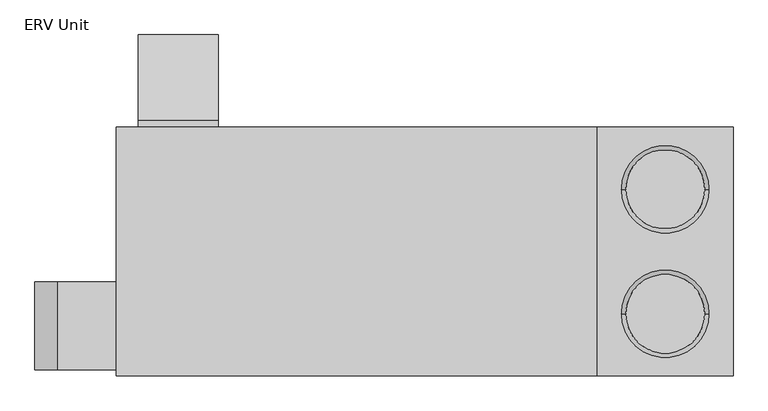
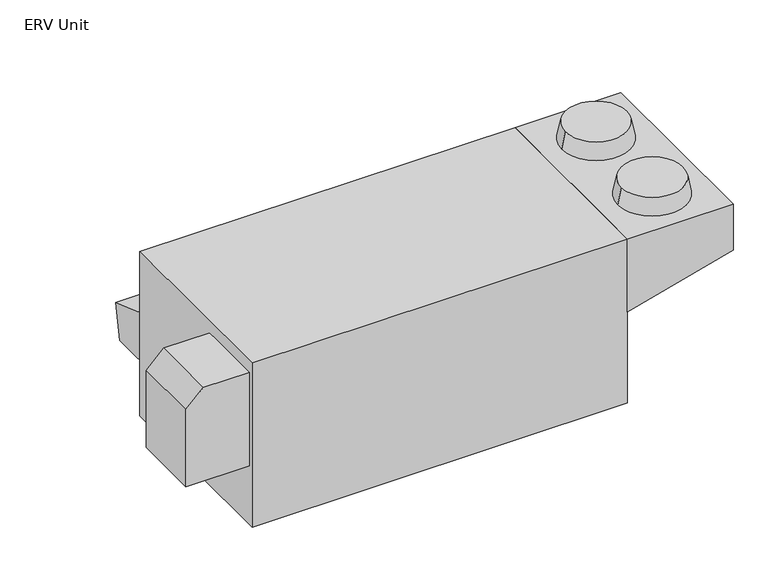
"""IFC4 building model written with IfcOpenShell, lengths in millimetres: proxy geometry, Energy Recovery-ER_H : ERV Unit."""

from ifc_helpers import new_model, si_unit, frame, origin, place, context, project, spatial, polyline, circle_curve, outline, extrude, source, transform, mapped, element, save
from ifc_brep_helpers import plane_surface, revolved_surface, advanced_brep


def erv_unit_62530c4e(model_context):
    return source(origin(), model_context, "Body", "SolidModel", [
        extrude(outline(polyline([(740.0249593, 200.025), (740.0249593, 635.0), (778.1249593, 635.0), (1267.0749593, 463.55), (1216.2749593, 200.025), (740.0249593, 200.025)])), frame((-44.3389519, 0.0, 0.0), z_axis=(1.0, 0.0, 0.0), x_axis=(0.0, 1.0, 0.0)), (0.0, 0.0, 1.0), 457.2),
        advanced_brep(
        [(3188.1285481, -326.7750407, 1346.2), (2736.6435481, -326.7750407, 1346.2), (3213.2110481, -326.7750407, 1219.2), (2711.5610481, -326.7750407, 1219.2)],
        [
            (0, 1, circle_curve(frame((2962.3860481, -326.7750407, 1346.2), z_axis=(0.0, 0.0, 1.0), x_axis=(1.0, 0.0, 0.0)), 225.7425)),
            (1, 0, circle_curve(frame((2962.3860481, -326.7750407, 1346.2), z_axis=(0.0, 0.0, 1.0), x_axis=(-1.0, 0.0, 0.0)), 225.7425)),
            (2, 3, circle_curve(frame((2962.3860481, -326.7750407, 1219.2), z_axis=(0.0, 0.0, -1.0), x_axis=(-1.0, 0.0, 0.0)), 250.825)),
            (3, 2, circle_curve(frame((2962.3860481, -326.7750407, 1219.2), z_axis=(0.0, 0.0, -1.0), x_axis=(1.0, 0.0, 0.0)), 250.825)),
            (3, 1),
            (0, 2),
        ],
        [
            plane_surface(frame((2962.3860481, -326.7750407, 1346.2), z_axis=(0.0, 0.0, 1.0), x_axis=(0.0, 1.0, 0.0))),
            plane_surface(frame((2962.3860481, -326.7750407, 1219.2), z_axis=(0.0, 0.0, -1.0), x_axis=(0.0, 1.0, 0.0))),
            revolved_surface(polyline([(3188.1285481, -326.7750407, 1346.2), (3213.2110481, -326.7750407, 1219.2)]), (2962.3860481, -326.7750407, 2489.2), (0.0, 0.0, -1.0)),
            revolved_surface(polyline([(2736.6435481, -326.7750407, 1346.2), (2711.5610481, -326.7750407, 1219.2)]), (2962.3860481, -326.7750407, 2489.2), (0.0, 0.0, -1.0)),
        ],
        [
            (0, [[1, 2]]),
            (1, [[3, 4]]),
            (2, [[-4, 5, -1, 6]]),
            (3, [[-3, -6, -2, -5]]),
        ],
    ),
        advanced_brep(
        [(3188.1285481, 384.4249593, 1346.2), (2736.6435481, 384.4249593, 1346.2), (3213.2110481, 384.4249593, 1219.2), (2711.5610481, 384.4249593, 1219.2)],
        [
            (0, 1, circle_curve(frame((2962.3860481, 384.4249593, 1346.2), z_axis=(0.0, 0.0, 1.0), x_axis=(1.0, 0.0, 0.0)), 225.7425)),
            (1, 0, circle_curve(frame((2962.3860481, 384.4249593, 1346.2), z_axis=(0.0, 0.0, 1.0), x_axis=(-1.0, 0.0, 0.0)), 225.7425)),
            (2, 3, circle_curve(frame((2962.3860481, 384.4249593, 1219.2), z_axis=(0.0, 0.0, -1.0), x_axis=(-1.0, 0.0, 0.0)), 250.825)),
            (3, 2, circle_curve(frame((2962.3860481, 384.4249593, 1219.2), z_axis=(0.0, 0.0, -1.0), x_axis=(1.0, 0.0, 0.0)), 250.825)),
            (3, 1),
            (0, 2),
        ],
        [
            plane_surface(frame((2962.3860481, 384.4249593, 1346.2), z_axis=(0.0, 0.0, 1.0), x_axis=(0.0, 1.0, 0.0))),
            plane_surface(frame((2962.3860481, 384.4249593, 1219.2), z_axis=(0.0, 0.0, -1.0), x_axis=(0.0, 1.0, 0.0))),
            revolved_surface(polyline([(3188.1285481, 384.4249593, 1346.2), (3213.2110481, 384.4249593, 1219.2)]), (2962.3860481, 384.4249593, 2489.2), (0.0, 0.0, -1.0)),
            revolved_surface(polyline([(2736.6435481, 384.4249593, 1346.2), (2711.5610481, 384.4249593, 1219.2)]), (2962.3860481, 384.4249593, 2489.2), (0.0, 0.0, -1.0)),
        ],
        [
            (0, [[1, 2]]),
            (1, [[3, 4]]),
            (2, [[-4, 5, -1, 6]]),
            (3, [[-3, -6, -2, -5]]),
        ],
    ),
        extrude(outline(polyline([(1219.2, 3349.7360481), (1219.2, 2575.0360481), (654.05, 2575.0360481), (863.6, 3349.7360481), (1219.2, 3349.7360481)])), frame((0.0, -682.3750407, 0.0), z_axis=(0.0, 1.0, 0.0), x_axis=(0.0, 0.0, 1.0)), (0.0, 0.0, 1.0), 1422.4),
        extrude(outline(polyline([(403.225, -171.3389519), (1127.125, -171.3389519), (1127.125, -507.8889519), (1000.125, -634.8889519), (403.225, -634.8889519), (403.225, -171.3389519)])), frame((0.0, -647.4500407, 0.0), z_axis=(0.0, 1.0, 0.0), x_axis=(0.0, 0.0, 1.0)), (0.0, 0.0, 1.0), 501.65),
        extrude(outline(polyline([(2060.6860481, 606.6749593), (2060.6860481, 276.4749593), (1425.6860481, 276.4749593), (1425.6860481, 606.6749593), (2060.6860481, 606.6749593)])), frame((0.0, 0.0, -50.8), z_axis=(0.0, 0.0, 1.0), x_axis=(1.0, 0.0, 0.0)), (0.0, 0.0, 1.0), 3.175),
        extrude(outline(polyline([(2194.0360481, -129.9250407), (2194.0360481, -587.1250407), (1838.4360481, -587.1250407), (1838.4360481, -129.9250407), (2194.0360481, -129.9250407)])), frame((0.0, 0.0, -50.8), z_axis=(0.0, 0.0, 1.0), x_axis=(1.0, 0.0, 0.0)), (0.0, 0.0, 1.0), 3.175),
        extrude(outline(polyline([(2575.0360481, 740.0249593), (2575.0360481, -682.3750407), (-171.3389519, -682.3750407), (-171.3389519, 740.0249593), (2575.0360481, 740.0249593)])), frame((0.0, 0.0, -50.8), z_axis=(0.0, 0.0, 1.0), x_axis=(1.0, 0.0, 0.0)), (0.0, 0.0, 1.0), 1270.0),
    ])


if __name__ == "__main__":
    model = new_model("IFC4")
    model_context = context("Model", 3, world=origin())
    ifc_project = project(units=[si_unit("LENGTHUNIT", "METRE", prefix="MILLI")], contexts=[model_context])
    site = spatial("IfcSite", under=ifc_project)
    building = spatial("IfcBuilding", under=site)
    placement = place(None, origin())
    erv_unit_shape = erv_unit_62530c4e(model_context)
    element("IfcBuildingElementProxy", 1, Name="Energy Recovery-ER_H : ERV Unit", ObjectType="Energy Recovery-ER_H : ERV Unit", at=placement, inside=building, context=model_context, shape_type="MappedRepresentation", body=[
        mapped(erv_unit_shape, transform((0.0, 0.0, 0.0), x_axis=(1.0, 0.0, 0.0), y_axis=(0.0, 1.0, 0.0), z_axis=(0.0, 0.0, 1.0))),
    ])
    save(model, "model.ifc")

# Revit data of these elements
# Type "Energy Recovery-ER_H : ERV Unit"
#   Version Family = "rfa 1.0 Beta"
#   Version Data = "NA"
#   URL = "http://www.greenheck.com/products/detail/51"
#   Tag = ""
#   Supply Filter = ""
#   OAI Weatherhood End Description = "Louvered Outdoor Air Intake"
#   OAI Duct Top Description = "Alternative connector is used"
#   OAI Duct End Description = "Alternative connector is used"
#   OAD Duct Top Description = "Alternative connector is used"
#   OAD Duct Side Description = "Alternative connector is used"
#   OAD Duct End Description = "Alternative connector is used"
#   OAD Duct Bottom Description = "Supply Air Discharge"
#   Model = "ERCH-20M-15"
#   Manufacturing Location = "United States"
#   Manufacturer = "Greenheck"
#   Invalid Connector = "Alternative connector is used"
#   Exhaust Filter = ""
#   Energy Wheel Model = "0"
#   EAI Duct Top Description = "Alternative connector is used"
#   EAI Duct Bottom Description = "Exhaust Air Intake"
#   EAI Duct Back Description = "Alternative connector is used"
#   EAD Weatherhood Side Description = "Side Exhaust Air Weatherhood"
#   EAD Weatherhood End Description = "Alternative connector is used"
#   EAD Duct Top Description = "Alternative connector is used"
#   EAD Duct Side Description = "Alternative connector is used"
#   EAD Duct End Description = "Alternative connector is used"
#   Description = "Energy Recovery with Cooling & Heating"
#   Copyright © = "© Greenheck Fan Corp 2009"
#   Configured Mark Name = "ERV Unit"
#   Voltage = 460 V
#   Unit Weight = 0.0000625 kip
#   Supply Static Pressure = 0.00 in-wg
#   Supply Air Flow Rate = 1400 CFM
#   PDX Length = 774.7 mm
#   PDX Front Height = 355.6 mm
#   PDX Cooling Radius Top = 225.743 mm
#   PDX Cooling Radius = 250.825 mm
#   PDX Back Height = 565.15 mm
#   OAI Half Depth = 231.775 mm
#   OAI Duct Width = 501.65 mm
#   OAI Duct Vert = 815.975 mm
#   OAI Duct Horiz = 285.75 mm
#   OAI Duct Height = 723.9 mm
#   OAI Depth = 463.55 mm
#   OAD Duct Width = 457.2 mm
#   OAD Duct Vert = 558.8 mm
#   OAD Duct Horiz = 323.85 mm
#   OAD Duct Height = 355.6 mm
#   Length PDX = 762 mm
#   IG Heater Width = 787.4 mm
#   IG Heater Offset = 25.4 mm
#   IG Heater Height = 0 mm
#   IG Heater Height NZ = 25.4 mm
#   IG Heater Depth = 254 mm
#   Half Under Sizing = 25.4 mm
#   Exhaust Static Pressure = 0.00 in-wg
#   Exhaust Air Flow Rate = 1400 CFM
#   Energy Wheel Depth = 38.1 mm
#   Electrical Load = 0 VA
#   Electrical Current = 60 Hz
#   EAI Duct Width = 330.2 mm
#   EAI Duct Vert = 831.85 mm
#   EAI Duct Horiz = 298.45 mm
#   EAI Duct Height = 635 mm
#   EAD Duct Width = 457.2 mm
#   EAD Duct Vert = 514.35 mm
#   EAD Duct Horiz = 355.6 mm
#   EAD Duct Height = 434.975 mm
#   EAD Depth = 527.05 mm
#   CurbWidth = 1371.6 mm
#   CurbLength = 2695.575 mm
#   Curb Under Sizing = 50.8 mm
#   Curb Height = 25.4 mm
#   Base Width = 1422.4 mm
#   Base Length = 2746.375 mm
#   Base Height = 1270 mm
#   VFD = no
#   Roof Curb = no
#   Phase = 3
#   Packaged DX = yes
#   OAI Weatherhood End = yes
#   OAI Duct Top = no
#   OAI Duct End = no
#   OAD Duct Top = no
#   OAD Duct Side = no
#   OAD Duct Bottom = yes
#   OAD Duct End = no
#   Number of Poles = 3
#   Indirect Gas Heater = yes
#   IG Heater Top = no
#   IG Heater Bottom = no
#   Has Special Design = no
#   EAI Duct Top = no
#   EAI Duct Bottom = yes
#   EAI Duct Back = no
#   EAD Weatherhood Side = yes
#   EAD Weatherhood End = no
#   EAD Duct Top = no
#   EAD Duct End = no
#   EAD Duct Side = no
#   Load Classification = HVAC
#   Type Comments = ""
#   Default Elevation = 0
#   Assembly Code = ""
